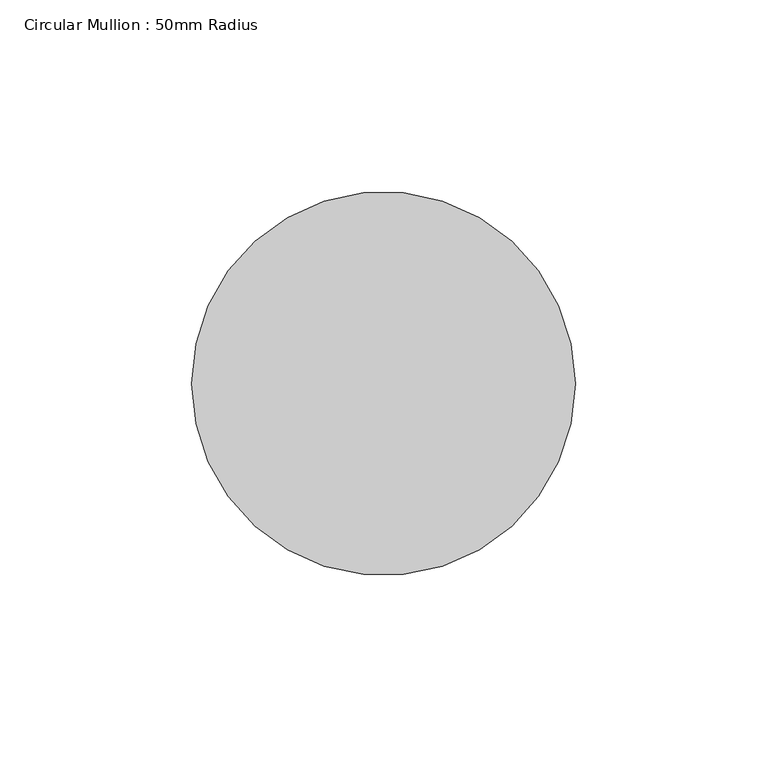
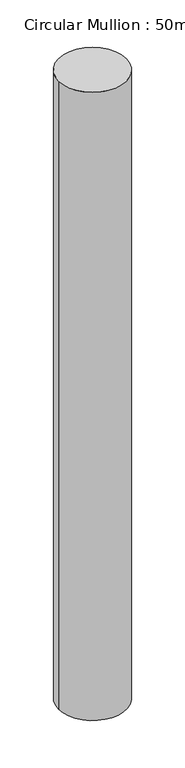
"""IFC4 building model written with IfcOpenShell, lengths in millimetres: member geometry, Circular Mullion : 50mm Radius."""

from ifc_helpers import new_model, si_unit, point, frame, origin, origin_2d, place, context, project, spatial, circle_curve, trimmed, segment, composite_curve, outline, extrude, source, transform, mapped, element, save


def circular_mullion_50mm_radius_e15ff7f8(model_context):
    return source(origin(), model_context, "Body", "SweptSolid", [
        extrude(outline(composite_curve([segment(trimmed(circle_curve(origin_2d(), 50.0), [point((50.0, 0.0))], [point((-50.0, 0.0))], False, "CARTESIAN"), True, "CONTINUOUS"), segment(trimmed(circle_curve(origin_2d(), 50.0), [point((-50.0, 0.0))], [point((50.0, 0.0))], False, "CARTESIAN"), True, "CONTINUOUS")], self_intersect=False)), frame((0.0, 0.0, -978.4433691), z_axis=(0.0, 0.0, 1.0), x_axis=(1.0, 0.0, 0.0)), (0.0, 0.0, 1.0), 978.4433691),
    ])


if __name__ == "__main__":
    model = new_model("IFC4")
    model_context = context("Model", 3, world=origin())
    ifc_project = project(units=[si_unit("LENGTHUNIT", "METRE", prefix="MILLI")], contexts=[model_context])
    site = spatial("IfcSite", under=ifc_project)
    building = spatial("IfcBuilding", under=site)
    placement = place(None, origin())
    circular_mullion_50mm_radius_shape = circular_mullion_50mm_radius_e15ff7f8(model_context)
    element("IfcMember", 1, ObjectType="Circular Mullion : 50mm Radius", at=placement, inside=building, context=model_context, shape_type="MappedRepresentation", body=[
        mapped(circular_mullion_50mm_radius_shape, transform((0.0, 0.0, 0.0), x_axis=(1.0, 0.0, 0.0), y_axis=(0.0, 1.0, 0.0), z_axis=(0.0, 0.0, 1.0))),
    ])
    save(model, "model.ifc")

# Revit data of these elements
# Type "Circular Mullion : 50mm Radius"
#   built-in parameter 1007350 = 0.164042 (stored number, unit not read)
# Element 1 (IfcMember, "Circular Mullion : 50mm Radius")
#   Materials on its faces: "Aluminium"
# Materials
#   "Aluminium": class "Metal", colour RGB 247 247 247, transparency 0, Description = "Aluminium 6061", Cost = 0
